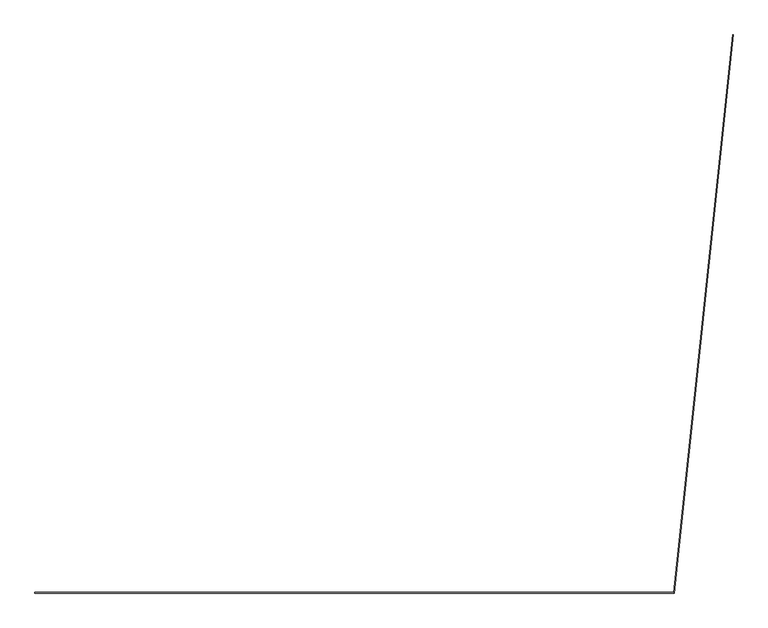
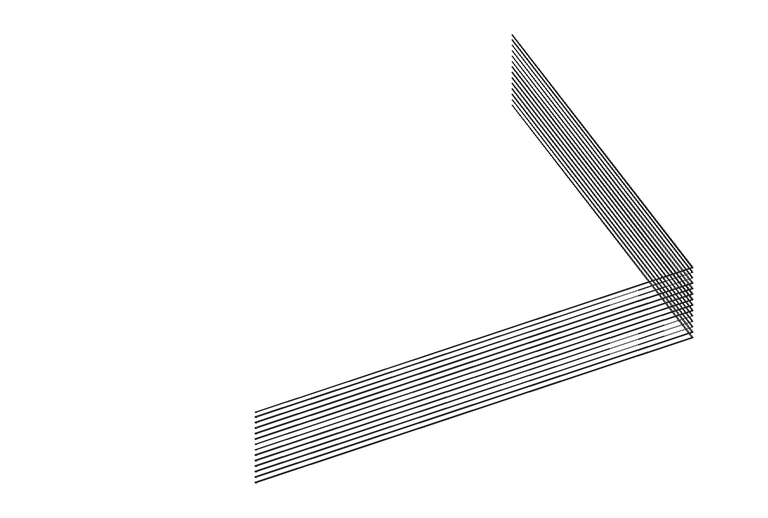
"""IFC4 building model written with IfcOpenShell, lengths in millimetres: railing geometry."""

import ifcopenshell
import ifcopenshell.guid

model = None  # the IFC model being written
_history = None  # IfcOwnerHistory: only IFC2X3 demands one
_inside = {}  # id of a spatial element -> (the spatial element, [elements in it])
_under = {}  # id of a project, library or spatial element -> (it, [spatial elements below it])
_declared = {}  # id of a project -> (the project, [libraries it declares])
_typed = {}  # id of a type object -> (the type object, [elements of that type])
_made_of = {}  # id of a material, layer set ... -> (it, [elements and type objects made of it])


def new_model(schema):
    """Start an empty IFC model of exactly this schema.

    Asked for "IFC4X3", IfcOpenShell would pick the latest addendum, in which some entities
    have other attributes; the version numbers below select the first issue.
    IFC2X3 requires an IfcOwnerHistory on every rooted entity: one is made here for all.
    """
    global model, _history
    if schema == "IFC4X3":
        model = ifcopenshell.file(schema_version=(4, 3, 0, 0))
    else:
        model = ifcopenshell.file(schema=schema)
    _inside.clear()
    _under.clear()
    _declared.clear()
    _typed.clear()
    _made_of.clear()
    _history = None
    if model.schema == "IFC2X3":
        org = make("IfcOrganization", Name="unknown")
        user = make(
            "IfcPersonAndOrganization",
            ThePerson=make("IfcPerson", FamilyName="unknown"),
            TheOrganization=org,
        )
        app = make(
            "IfcApplication",
            ApplicationDeveloper=org,
            Version="unknown",
            ApplicationFullName="unknown",
            ApplicationIdentifier="unknown",
        )
        _history = make(
            "IfcOwnerHistory",
            OwningUser=user,
            OwningApplication=app,
            ChangeAction="ADDED",
            CreationDate=0,
        )
    return model


def make(cls, **values):
    """One entity of the class cls with the attributes given. An attribute that is None is left unset."""
    return model.create_entity(
        cls, **{name: value for name, value in values.items() if value is not None}
    )


def rooted(cls, **values):
    """An entity with a GlobalId (a new one), such as an element, a storey or a relation."""
    return make(cls, GlobalId=ifcopenshell.guid.new(), OwnerHistory=_history, **values)


def si_unit(unit_type, name, prefix=None):
    """IfcSIUnit, for example si_unit("LENGTHUNIT", "METRE", prefix="MILLI")."""
    return make("IfcSIUnit", UnitType=unit_type, Prefix=prefix, Name=name)


def assignment(units):
    """IfcUnitAssignment: the units of a project."""
    return None if units is None else make("IfcUnitAssignment", Units=units)


def point(xyz):
    """IfcCartesianPoint."""
    return None if xyz is None else make("IfcCartesianPoint", Coordinates=xyz)


def direction(xyz):
    """IfcDirection."""
    return None if xyz is None else make("IfcDirection", DirectionRatios=xyz)


def frame(location, z_axis=None, x_axis=None):
    """IfcAxis2Placement3D, a coordinate frame: its origin and axes. An axis left out is left unset."""
    return make(
        "IfcAxis2Placement3D",
        Location=point(location),
        Axis=direction(z_axis),
        RefDirection=direction(x_axis),
    )


def origin():
    """The frame at (0, 0, 0) with its axes left unset."""
    return frame((0.0, 0.0, 0.0))


def place(relative_to, where):
    """IfcLocalPlacement: puts the frame where relative to a parent placement (None: the world)."""
    return make(
        "IfcLocalPlacement", PlacementRelTo=relative_to, RelativePlacement=where
    )


def context(
    kind, dimensions, precision=None, world=None, true_north=None, identifier=None
):
    """IfcGeometricRepresentationContext, for example the 3D "Model" context."""
    return make(
        "IfcGeometricRepresentationContext",
        ContextIdentifier=identifier,
        ContextType=kind,
        CoordinateSpaceDimension=dimensions,
        Precision=precision,
        WorldCoordinateSystem=world,
        TrueNorth=true_north,
    )


def project(units=None, contexts=None):
    """IfcProject with its units and contexts."""
    return rooted(
        "IfcProject",
        Name="project",
        RepresentationContexts=contexts,
        UnitsInContext=assignment(units),
    )


def spatial(cls, under=None, at=None, **own):
    """A site, building, storey or space (cls), placed at a placement, below another one or the project."""
    s = rooted(cls, ObjectPlacement=at, **own)
    if under is not None:
        _under.setdefault(under.id(), (under, []))[1].append(s)
    return s


def circle_curve(where, radius):
    """IfcCircle in the frame where."""
    return make("IfcCircle", Position=where, Radius=radius)


def ellipse_curve(where, semi_axis1, semi_axis2):
    """IfcEllipse in the frame where."""
    return make(
        "IfcEllipse", Position=where, SemiAxis1=semi_axis1, SemiAxis2=semi_axis2
    )


def shape(context_of_items, identifier, shape_type, items):
    """IfcShapeRepresentation: the items that make up one representation, for example the "Body"."""
    return make(
        "IfcShapeRepresentation",
        ContextOfItems=context_of_items,
        RepresentationIdentifier=identifier,
        RepresentationType=shape_type,
        Items=items,
    )


def source(mapping_origin, context_of_items, identifier, shape_type, items):
    """IfcRepresentationMap: a shape defined once, which mapped items show again and again."""
    return make(
        "IfcRepresentationMap",
        MappingOrigin=mapping_origin,
        MappedRepresentation=shape(context_of_items, identifier, shape_type, items),
    )


def transform(
    local_origin,
    x_axis=None,
    y_axis=None,
    z_axis=None,
    scale=None,
    scale2=None,
    scale3=None,
    uniform=True,
):
    """IfcCartesianTransformationOperator3D, or its non-uniform kind. x_axis, y_axis, z_axis: its Axis1, 2, 3."""
    if uniform:
        return make(
            "IfcCartesianTransformationOperator3D",
            Axis1=direction(x_axis),
            Axis2=direction(y_axis),
            LocalOrigin=point(local_origin),
            Scale=scale,
            Axis3=direction(z_axis),
        )
    return make(
        "IfcCartesianTransformationOperator3DnonUniform",
        Axis1=direction(x_axis),
        Axis2=direction(y_axis),
        LocalOrigin=point(local_origin),
        Scale=scale,
        Axis3=direction(z_axis),
        Scale2=scale2,
        Scale3=scale3,
    )


def mapped(mapping_source, mapping_target):
    """IfcMappedItem: shows the shape of a source again, moved by a transform."""
    return make(
        "IfcMappedItem", MappingSource=mapping_source, MappingTarget=mapping_target
    )


def made_of(thing, what):
    """Note that an element or type object is made of a material, layer set ...; save() writes the relation."""
    if what is not None:
        _made_of.setdefault(what.id(), (what, []))[1].append(thing)
    return thing


def element(
    cls,
    number,
    at=None,
    inside=None,
    cuts=None,
    type_object=None,
    material=None,
    context=None,
    identifier="Body",
    shape_type=None,
    held_by="IfcProductDefinitionShape",
    body=None,
    shapes=None,
    **own,
):
    """One element of the class cls, such as IfcWall. Its Tag is "e" and its number.

    at: its placement. inside: the storey or other place that contains it. cuts: it is an
    opening in that element (IfcRelVoidsElement). A single representation is given by context,
    identifier, shape_type and body (its items); several are given by shapes. held_by: the class
    of the entity that holds the representations. save() writes the other relations.
    """
    e = rooted(cls, Tag="e%d" % number, ObjectPlacement=at, **own)
    if body is not None:
        shapes = [shape(context, identifier, shape_type, body)]
    if shapes is not None:
        e.Representation = make(held_by, Representations=shapes)
    if inside is not None:
        _inside.setdefault(inside.id(), (inside, []))[1].append(e)
    if cuts is not None:
        rooted(
            "IfcRelVoidsElement", RelatingBuildingElement=cuts, RelatedOpeningElement=e
        )
    if type_object is not None:
        _typed.setdefault(type_object.id(), (type_object, []))[1].append(e)
    return made_of(e, material)


def aggregate(whole, parts):
    """IfcRelAggregates: a whole, such as a stair, and the parts it consists of."""
    return rooted("IfcRelAggregates", RelatingObject=whole, RelatedObjects=parts)


def save(model, path):
    """Write the relations noted so far, then the file.

    IfcRelAggregates (storeys below a building ...), IfcRelContainedInSpatialStructure (elements
    in a storey), IfcRelDefinesByType, IfcRelAssociatesMaterial and IfcRelDeclares: one each for
    every whole, place, type object, material and project.
    """
    for whole, parts in _under.values():
        aggregate(whole, parts)
    for where, things in _inside.values():
        rooted(
            "IfcRelContainedInSpatialStructure",
            RelatedElements=things,
            RelatingStructure=where,
        )
    for kind, things in _typed.values():
        rooted("IfcRelDefinesByType", RelatedObjects=things, RelatingType=kind)
    for what, things in _made_of.values():
        rooted("IfcRelAssociatesMaterial", RelatedObjects=things, RelatingMaterial=what)
    for by, libraries in _declared.values():
        rooted("IfcRelDeclares", RelatingContext=by, RelatedDefinitions=libraries)
    model.write(path)


def plane_surface(at):
    """IfcPlane: the flat surface through the origin of the frame at, square to its z axis."""
    return make("IfcPlane", Position=at)


def cylinder_surface(at, radius):
    """IfcCylindricalSurface: all points at the distance radius from the z axis of the frame at."""
    return make("IfcCylindricalSurface", Position=at, Radius=radius)


def advanced_brep(points, edges, surfaces, faces):
    """IfcAdvancedBrep: a solid bounded by faces that lie on surfaces and meet in shared edges.

    An edge is (start, end): straight between two places in points (the first is 0);
    or (start, end, curve); or (start, end, curve, False) where it runs against its curve.
    A face is (place in surfaces, loops), or (place, loops, False) where it looks against
    its surface's normal. A loop lists edges by number (the first is 1), with a minus sign
    where the edge is run from its end to its start. The first loop is the outer one.
    """
    corners = [point(p) for p in points]
    vertices = [make("IfcVertexPoint", VertexGeometry=c) for c in corners]
    made = []
    for start, end, *more in edges:
        made.append(
            make(
                "IfcEdgeCurve",
                EdgeStart=vertices[start],
                EdgeEnd=vertices[end],
                EdgeGeometry=more[0] if more else make("IfcPolyline", Points=[corners[start], corners[end]]),
                SameSense=more[1] if len(more) > 1 else True,
            )
        )
    hull = []
    for where, loops, *sense in faces:
        bounds = []
        for j, loop in enumerate(loops):
            ring = [make("IfcOrientedEdge", EdgeElement=made[abs(k) - 1], Orientation=k > 0) for k in loop]
            bounds.append(
                make(
                    "IfcFaceOuterBound" if j == 0 else "IfcFaceBound",
                    Bound=make("IfcEdgeLoop", EdgeList=ring),
                    Orientation=True,
                )
            )
        hull.append(make("IfcAdvancedFace", Bounds=bounds, FaceSurface=surfaces[where], SameSense=sense[0] if sense else True))
    return make("IfcAdvancedBrep", Outer=make("IfcClosedShell", CfsFaces=hull))


def railing_c9f429d1(model_context):
    return source(origin(), model_context, "Body", "AdvancedBrep", [
        advanced_brep(
        [(34239.1491327, 30677.9041051, 270256.79375), (34234.4127222, 30678.4019219, 270256.79375), (27919.3590778, 25622.1094112, 270256.79375), (27919.3590778, 25626.8719112, 270256.79375), (33707.7636978, 25622.1094112, 270256.79375), (33703.4755235, 25626.8719112, 270256.79375)],
        [
            (0, 1, circle_curve(frame((34236.7809275, 30678.1530135, 270256.79375), z_axis=(0.10452846326765991, 0.9945218953682727, 0.0), x_axis=(-0.9945218953682727, 0.10452846326765991, 0.0)), 2.38125)),
            (1, 0, circle_curve(frame((34236.7809275, 30678.1530135, 270256.79375), z_axis=(0.10452846326765991, 0.9945218953682727, 0.0), x_axis=(-0.9945218953682727, 0.10452846326765991, 0.0)), 2.38125)),
            (2, 3, circle_curve(frame((27919.3590778, 25624.4906612, 270256.79375), z_axis=(-1.0, 0.0, 0.0), x_axis=(0.0, 1.0, 0.0)), 2.38125)),
            (3, 2, circle_curve(frame((27919.3590778, 25624.4906612, 270256.79375), z_axis=(-1.0, 0.0, 0.0), x_axis=(0.0, 1.0, 0.0)), 2.38125)),
            (0, 4),
            (4, 5, ellipse_curve(frame((33705.6196106, 25624.4906612, 270256.79375), z_axis=(0.7431448254773977, 0.6691306063588546, 0.0), x_axis=(-0.6691306063588546, 0.7431448254773974, 0.0)), 3.2042879, 2.38125)),
            (5, 1),
            (5, 4, ellipse_curve(frame((33705.6196106, 25624.4906612, 270256.79375), z_axis=(0.7431448254773977, 0.6691306063588546, 0.0), x_axis=(-0.6691306063588546, 0.7431448254773974, 0.0)), 3.2042879, 2.38125)),
            (4, 2),
            (3, 5),
        ],
        [
            plane_surface(frame((34236.7809275, 30678.1530135, 270259.175), z_axis=(0.10452846326765991, 0.9945218953682727, 0.0), x_axis=(0.9945218953682727, -0.10452846326765991, 0.0))),
            plane_surface(frame((27919.3590778, 25624.4906612, 270259.175), z_axis=(-1.0, 0.0, 0.0), x_axis=(0.0, -1.0, 0.0))),
            cylinder_surface(frame((34236.7809275, 30678.1530135, 270256.79375), z_axis=(0.10452846326765991, 0.9945218953682727, 0.0), x_axis=(-0.9945218953682727, 0.10452846326765991, 0.0)), 2.38125),
            cylinder_surface(frame((33705.6196106, 25624.4906612, 270256.79375), z_axis=(1.0, 0.0, 0.0), x_axis=(0.0, 1.0, 0.0)), 2.38125),
        ],
        [
            (0, [[1, 2]]),
            (1, [[3, 4]]),
            (2, [[-1, 5, 6, 7]]),
            (2, [[-2, -7, 8, -5]]),
            (3, [[-6, 9, -4, 10]]),
            (3, [[-8, -10, -3, -9]]),
        ],
    ),
        advanced_brep(
        [(34239.1491327, 30677.9041051, 270190.11875), (34234.4127222, 30678.4019219, 270190.11875), (33707.7636978, 25622.1094112, 270190.11875), (33703.4755235, 25626.8719112, 270190.11875), (27919.3590778, 25622.1094112, 270190.11875), (27919.3590778, 25626.8719112, 270190.11875)],
        [
            (0, 1, circle_curve(frame((34236.7809275, 30678.1530135, 270190.11875), z_axis=(0.10452846326765991, 0.9945218953682727, 0.0), x_axis=(-0.9945218953682727, 0.10452846326765991, 0.0)), 2.38125)),
            (1, 0, circle_curve(frame((34236.7809275, 30678.1530135, 270190.11875), z_axis=(0.10452846326765991, 0.9945218953682727, 0.0), x_axis=(-0.9945218953682727, 0.10452846326765991, 0.0)), 2.38125)),
            (0, 2),
            (2, 3, ellipse_curve(frame((33705.6196106, 25624.4906612, 270190.11875), z_axis=(0.7431448254773977, 0.6691306063588546, 0.0), x_axis=(-0.6691306063588546, 0.7431448254773974, 0.0)), 3.2042879, 2.38125)),
            (3, 1),
            (3, 2, ellipse_curve(frame((33705.6196106, 25624.4906612, 270190.11875), z_axis=(0.7431448254773977, 0.6691306063588546, 0.0), x_axis=(-0.6691306063588546, 0.7431448254773974, 0.0)), 3.2042879, 2.38125)),
            (4, 5, circle_curve(frame((27919.3590778, 25624.4906612, 270190.11875), z_axis=(-1.0, 0.0, 0.0), x_axis=(0.0, 1.0, 0.0)), 2.38125)),
            (5, 4, circle_curve(frame((27919.3590778, 25624.4906612, 270190.11875), z_axis=(-1.0, 0.0, 0.0), x_axis=(0.0, 1.0, 0.0)), 2.38125)),
            (2, 4),
            (5, 3),
        ],
        [
            plane_surface(frame((34236.7809275, 30678.1530135, 270192.5), z_axis=(0.10452846326765991, 0.9945218953682727, 0.0), x_axis=(0.9945218953682727, -0.10452846326765991, 0.0))),
            cylinder_surface(frame((34236.7809275, 30678.1530135, 270190.11875), z_axis=(0.10452846326765991, 0.9945218953682727, 0.0), x_axis=(-0.9945218953682727, 0.10452846326765991, 0.0)), 2.38125),
            plane_surface(frame((27919.3590778, 25624.4906612, 270192.5), z_axis=(-1.0, 0.0, 0.0), x_axis=(0.0, -1.0, 0.0))),
            cylinder_surface(frame((33705.6196106, 25624.4906612, 270190.11875), z_axis=(1.0, 0.0, 0.0), x_axis=(0.0, 1.0, 0.0)), 2.38125),
        ],
        [
            (0, [[1, 2]]),
            (1, [[-1, 3, 4, 5]]),
            (1, [[-2, -5, 6, -3]]),
            (2, [[7, 8]]),
            (3, [[-4, 9, -8, 10]]),
            (3, [[-6, -10, -7, -9]]),
        ],
    ),
        advanced_brep(
        [(34239.1491327, 30677.9041051, 270113.91875), (34234.4127222, 30678.4019219, 270113.91875), (33707.7636978, 25622.1094112, 270113.91875), (33703.4755235, 25626.8719112, 270113.91875), (27919.3590778, 25622.1094112, 270113.91875), (27919.3590778, 25626.8719112, 270113.91875)],
        [
            (0, 1, circle_curve(frame((34236.7809275, 30678.1530135, 270113.91875), z_axis=(0.10452846326765991, 0.9945218953682727, 0.0), x_axis=(-0.9945218953682727, 0.10452846326765991, 0.0)), 2.38125)),
            (1, 0, circle_curve(frame((34236.7809275, 30678.1530135, 270113.91875), z_axis=(0.10452846326765991, 0.9945218953682727, 0.0), x_axis=(-0.9945218953682727, 0.10452846326765991, 0.0)), 2.38125)),
            (0, 2),
            (2, 3, ellipse_curve(frame((33705.6196106, 25624.4906612, 270113.91875), z_axis=(0.7431448254773977, 0.6691306063588546, 0.0), x_axis=(-0.6691306063588546, 0.7431448254773974, 0.0)), 3.2042879, 2.38125)),
            (3, 1),
            (3, 2, ellipse_curve(frame((33705.6196106, 25624.4906612, 270113.91875), z_axis=(0.7431448254773977, 0.6691306063588546, 0.0), x_axis=(-0.6691306063588546, 0.7431448254773974, 0.0)), 3.2042879, 2.38125)),
            (4, 5, circle_curve(frame((27919.3590778, 25624.4906612, 270113.91875), z_axis=(-1.0, 0.0, 0.0), x_axis=(0.0, 1.0, 0.0)), 2.38125)),
            (5, 4, circle_curve(frame((27919.3590778, 25624.4906612, 270113.91875), z_axis=(-1.0, 0.0, 0.0), x_axis=(0.0, 1.0, 0.0)), 2.38125)),
            (2, 4),
            (5, 3),
        ],
        [
            plane_surface(frame((34236.7809275, 30678.1530135, 270116.3), z_axis=(0.10452846326765991, 0.9945218953682727, 0.0), x_axis=(0.9945218953682727, -0.10452846326765991, 0.0))),
            cylinder_surface(frame((34236.7809275, 30678.1530135, 270113.91875), z_axis=(0.10452846326765991, 0.9945218953682727, 0.0), x_axis=(-0.9945218953682727, 0.10452846326765991, 0.0)), 2.38125),
            plane_surface(frame((27919.3590778, 25624.4906612, 270116.3), z_axis=(-1.0, 0.0, 0.0), x_axis=(0.0, -1.0, 0.0))),
            cylinder_surface(frame((33705.6196106, 25624.4906612, 270113.91875), z_axis=(1.0, 0.0, 0.0), x_axis=(0.0, 1.0, 0.0)), 2.38125),
        ],
        [
            (0, [[1, 2]]),
            (1, [[-1, 3, 4, 5]]),
            (1, [[-2, -5, 6, -3]]),
            (2, [[7, 8]]),
            (3, [[-4, 9, -8, 10]]),
            (3, [[-6, -10, -7, -9]]),
        ],
    ),
        advanced_brep(
        [(34239.1491327, 30677.9041051, 270037.71875), (34234.4127222, 30678.4019219, 270037.71875), (33707.7636978, 25622.1094112, 270037.71875), (33703.4755235, 25626.8719112, 270037.71875), (27919.3590778, 25622.1094112, 270037.71875), (27919.3590778, 25626.8719112, 270037.71875)],
        [
            (0, 1, circle_curve(frame((34236.7809275, 30678.1530135, 270037.71875), z_axis=(0.10452846326765991, 0.9945218953682727, 0.0), x_axis=(-0.9945218953682727, 0.10452846326765991, 0.0)), 2.38125)),
            (1, 0, circle_curve(frame((34236.7809275, 30678.1530135, 270037.71875), z_axis=(0.10452846326765991, 0.9945218953682727, 0.0), x_axis=(-0.9945218953682727, 0.10452846326765991, 0.0)), 2.38125)),
            (0, 2),
            (2, 3, ellipse_curve(frame((33705.6196106, 25624.4906612, 270037.71875), z_axis=(0.7431448254773977, 0.6691306063588546, 0.0), x_axis=(-0.6691306063588546, 0.7431448254773974, 0.0)), 3.2042879, 2.38125)),
            (3, 1),
            (3, 2, ellipse_curve(frame((33705.6196106, 25624.4906612, 270037.71875), z_axis=(0.7431448254773977, 0.6691306063588546, 0.0), x_axis=(-0.6691306063588546, 0.7431448254773974, 0.0)), 3.2042879, 2.38125)),
            (4, 5, circle_curve(frame((27919.3590778, 25624.4906612, 270037.71875), z_axis=(-1.0, 0.0, 0.0), x_axis=(0.0, 1.0, 0.0)), 2.38125)),
            (5, 4, circle_curve(frame((27919.3590778, 25624.4906612, 270037.71875), z_axis=(-1.0, 0.0, 0.0), x_axis=(0.0, 1.0, 0.0)), 2.38125)),
            (2, 4),
            (5, 3),
        ],
        [
            plane_surface(frame((34236.7809275, 30678.1530135, 270040.1), z_axis=(0.10452846326765991, 0.9945218953682727, 0.0), x_axis=(0.9945218953682727, -0.10452846326765991, 0.0))),
            cylinder_surface(frame((34236.7809275, 30678.1530135, 270037.71875), z_axis=(0.10452846326765991, 0.9945218953682727, 0.0), x_axis=(-0.9945218953682727, 0.10452846326765991, 0.0)), 2.38125),
            plane_surface(frame((27919.3590778, 25624.4906612, 270040.1), z_axis=(-1.0, 0.0, 0.0), x_axis=(0.0, -1.0, 0.0))),
            cylinder_surface(frame((33705.6196106, 25624.4906612, 270037.71875), z_axis=(1.0, 0.0, 0.0), x_axis=(0.0, 1.0, 0.0)), 2.38125),
        ],
        [
            (0, [[1, 2]]),
            (1, [[-1, 3, 4, 5]]),
            (1, [[-2, -5, 6, -3]]),
            (2, [[7, 8]]),
            (3, [[-4, 9, -8, 10]]),
            (3, [[-6, -10, -7, -9]]),
        ],
    ),
        advanced_brep(
        [(34239.1491327, 30677.9041051, 269961.51875), (34234.4127222, 30678.4019219, 269961.51875), (33707.7636978, 25622.1094112, 269961.51875), (33703.4755235, 25626.8719112, 269961.51875), (27919.3590778, 25622.1094112, 269961.51875), (27919.3590778, 25626.8719112, 269961.51875)],
        [
            (0, 1, circle_curve(frame((34236.7809275, 30678.1530135, 269961.51875), z_axis=(0.10452846326765991, 0.9945218953682727, 0.0), x_axis=(-0.9945218953682727, 0.10452846326765991, 0.0)), 2.38125)),
            (1, 0, circle_curve(frame((34236.7809275, 30678.1530135, 269961.51875), z_axis=(0.10452846326765991, 0.9945218953682727, 0.0), x_axis=(-0.9945218953682727, 0.10452846326765991, 0.0)), 2.38125)),
            (0, 2),
            (2, 3, ellipse_curve(frame((33705.6196106, 25624.4906612, 269961.51875), z_axis=(0.7431448254773977, 0.6691306063588546, 0.0), x_axis=(-0.6691306063588546, 0.7431448254773974, 0.0)), 3.2042879, 2.38125)),
            (3, 1),
            (3, 2, ellipse_curve(frame((33705.6196106, 25624.4906612, 269961.51875), z_axis=(0.7431448254773977, 0.6691306063588546, 0.0), x_axis=(-0.6691306063588546, 0.7431448254773974, 0.0)), 3.2042879, 2.38125)),
            (4, 5, circle_curve(frame((27919.3590778, 25624.4906612, 269961.51875), z_axis=(-1.0, 0.0, 0.0), x_axis=(0.0, 1.0, 0.0)), 2.38125)),
            (5, 4, circle_curve(frame((27919.3590778, 25624.4906612, 269961.51875), z_axis=(-1.0, 0.0, 0.0), x_axis=(0.0, 1.0, 0.0)), 2.38125)),
            (2, 4),
            (5, 3),
        ],
        [
            plane_surface(frame((34236.7809275, 30678.1530135, 269963.9), z_axis=(0.10452846326765991, 0.9945218953682727, 0.0), x_axis=(0.9945218953682727, -0.10452846326765991, 0.0))),
            cylinder_surface(frame((34236.7809275, 30678.1530135, 269961.51875), z_axis=(0.10452846326765991, 0.9945218953682727, 0.0), x_axis=(-0.9945218953682727, 0.10452846326765991, 0.0)), 2.38125),
            plane_surface(frame((27919.3590778, 25624.4906612, 269963.9), z_axis=(-1.0, 0.0, 0.0), x_axis=(0.0, -1.0, 0.0))),
            cylinder_surface(frame((33705.6196106, 25624.4906612, 269961.51875), z_axis=(1.0, 0.0, 0.0), x_axis=(0.0, 1.0, 0.0)), 2.38125),
        ],
        [
            (0, [[1, 2]]),
            (1, [[-1, 3, 4, 5]]),
            (1, [[-2, -5, 6, -3]]),
            (2, [[7, 8]]),
            (3, [[-4, 9, -8, 10]]),
            (3, [[-6, -10, -7, -9]]),
        ],
    ),
        advanced_brep(
        [(34239.1491327, 30677.9041051, 269885.31875), (34234.4127222, 30678.4019219, 269885.31875), (33707.7636978, 25622.1094112, 269885.31875), (33703.4755235, 25626.8719112, 269885.31875), (27919.3590778, 25622.1094112, 269885.31875), (27919.3590778, 25626.8719112, 269885.31875)],
        [
            (0, 1, circle_curve(frame((34236.7809275, 30678.1530135, 269885.31875), z_axis=(0.10452846326765991, 0.9945218953682727, 0.0), x_axis=(-0.9945218953682727, 0.10452846326765991, 0.0)), 2.38125)),
            (1, 0, circle_curve(frame((34236.7809275, 30678.1530135, 269885.31875), z_axis=(0.10452846326765991, 0.9945218953682727, 0.0), x_axis=(-0.9945218953682727, 0.10452846326765991, 0.0)), 2.38125)),
            (0, 2),
            (2, 3, ellipse_curve(frame((33705.6196106, 25624.4906612, 269885.31875), z_axis=(0.7431448254773977, 0.6691306063588546, 0.0), x_axis=(-0.6691306063588546, 0.7431448254773974, 0.0)), 3.2042879, 2.38125)),
            (3, 1),
            (3, 2, ellipse_curve(frame((33705.6196106, 25624.4906612, 269885.31875), z_axis=(0.7431448254773977, 0.6691306063588546, 0.0), x_axis=(-0.6691306063588546, 0.7431448254773974, 0.0)), 3.2042879, 2.38125)),
            (4, 5, circle_curve(frame((27919.3590778, 25624.4906612, 269885.31875), z_axis=(-1.0, 0.0, 0.0), x_axis=(0.0, 1.0, 0.0)), 2.38125)),
            (5, 4, circle_curve(frame((27919.3590778, 25624.4906612, 269885.31875), z_axis=(-1.0, 0.0, 0.0), x_axis=(0.0, 1.0, 0.0)), 2.38125)),
            (2, 4),
            (5, 3),
        ],
        [
            plane_surface(frame((34236.7809275, 30678.1530135, 269887.7), z_axis=(0.10452846326765991, 0.9945218953682727, 0.0), x_axis=(0.9945218953682727, -0.10452846326765991, 0.0))),
            cylinder_surface(frame((34236.7809275, 30678.1530135, 269885.31875), z_axis=(0.10452846326765991, 0.9945218953682727, 0.0), x_axis=(-0.9945218953682727, 0.10452846326765991, 0.0)), 2.38125),
            plane_surface(frame((27919.3590778, 25624.4906612, 269887.7), z_axis=(-1.0, 0.0, 0.0), x_axis=(0.0, -1.0, 0.0))),
            cylinder_surface(frame((33705.6196106, 25624.4906612, 269885.31875), z_axis=(1.0, 0.0, 0.0), x_axis=(0.0, 1.0, 0.0)), 2.38125),
        ],
        [
            (0, [[1, 2]]),
            (1, [[-1, 3, 4, 5]]),
            (1, [[-2, -5, 6, -3]]),
            (2, [[7, 8]]),
            (3, [[-4, 9, -8, 10]]),
            (3, [[-6, -10, -7, -9]]),
        ],
    ),
        advanced_brep(
        [(34239.1491327, 30677.9041051, 269809.11875), (34234.4127222, 30678.4019219, 269809.11875), (33707.7636978, 25622.1094112, 269809.11875), (33703.4755235, 25626.8719112, 269809.11875), (27919.3590778, 25622.1094112, 269809.11875), (27919.3590778, 25626.8719112, 269809.11875)],
        [
            (0, 1, circle_curve(frame((34236.7809275, 30678.1530135, 269809.11875), z_axis=(0.10452846326765991, 0.9945218953682727, 0.0), x_axis=(-0.9945218953682727, 0.10452846326765991, 0.0)), 2.38125)),
            (1, 0, circle_curve(frame((34236.7809275, 30678.1530135, 269809.11875), z_axis=(0.10452846326765991, 0.9945218953682727, 0.0), x_axis=(-0.9945218953682727, 0.10452846326765991, 0.0)), 2.38125)),
            (0, 2),
            (2, 3, ellipse_curve(frame((33705.6196106, 25624.4906612, 269809.11875), z_axis=(0.7431448254773977, 0.6691306063588546, 0.0), x_axis=(-0.6691306063588546, 0.7431448254773974, 0.0)), 3.2042879, 2.38125)),
            (3, 1),
            (3, 2, ellipse_curve(frame((33705.6196106, 25624.4906612, 269809.11875), z_axis=(0.7431448254773977, 0.6691306063588546, 0.0), x_axis=(-0.6691306063588546, 0.7431448254773974, 0.0)), 3.2042879, 2.38125)),
            (4, 5, circle_curve(frame((27919.3590778, 25624.4906612, 269809.11875), z_axis=(-1.0, 0.0, 0.0), x_axis=(0.0, 1.0, 0.0)), 2.38125)),
            (5, 4, circle_curve(frame((27919.3590778, 25624.4906612, 269809.11875), z_axis=(-1.0, 0.0, 0.0), x_axis=(0.0, 1.0, 0.0)), 2.38125)),
            (2, 4),
            (5, 3),
        ],
        [
            plane_surface(frame((34236.7809275, 30678.1530135, 269811.5), z_axis=(0.10452846326765991, 0.9945218953682727, 0.0), x_axis=(0.9945218953682727, -0.10452846326765991, 0.0))),
            cylinder_surface(frame((34236.7809275, 30678.1530135, 269809.11875), z_axis=(0.10452846326765991, 0.9945218953682727, 0.0), x_axis=(-0.9945218953682727, 0.10452846326765991, 0.0)), 2.38125),
            plane_surface(frame((27919.3590778, 25624.4906612, 269811.5), z_axis=(-1.0, 0.0, 0.0), x_axis=(0.0, -1.0, 0.0))),
            cylinder_surface(frame((33705.6196106, 25624.4906612, 269809.11875), z_axis=(1.0, 0.0, 0.0), x_axis=(0.0, 1.0, 0.0)), 2.38125),
        ],
        [
            (0, [[1, 2]]),
            (1, [[-1, 3, 4, 5]]),
            (1, [[-2, -5, 6, -3]]),
            (2, [[7, 8]]),
            (3, [[-4, 9, -8, 10]]),
            (3, [[-6, -10, -7, -9]]),
        ],
    ),
        advanced_brep(
        [(34239.1491327, 30677.9041051, 269732.91875), (34234.4127222, 30678.4019219, 269732.91875), (33707.7636978, 25622.1094112, 269732.91875), (33703.4755235, 25626.8719112, 269732.91875), (27919.3590778, 25622.1094112, 269732.91875), (27919.3590778, 25626.8719112, 269732.91875)],
        [
            (0, 1, circle_curve(frame((34236.7809275, 30678.1530135, 269732.91875), z_axis=(0.10452846326765991, 0.9945218953682727, 0.0), x_axis=(-0.9945218953682727, 0.10452846326765991, 0.0)), 2.38125)),
            (1, 0, circle_curve(frame((34236.7809275, 30678.1530135, 269732.91875), z_axis=(0.10452846326765991, 0.9945218953682727, 0.0), x_axis=(-0.9945218953682727, 0.10452846326765991, 0.0)), 2.38125)),
            (0, 2),
            (2, 3, ellipse_curve(frame((33705.6196106, 25624.4906612, 269732.91875), z_axis=(0.7431448254773977, 0.6691306063588546, 0.0), x_axis=(-0.6691306063588546, 0.7431448254773974, 0.0)), 3.2042879, 2.38125)),
            (3, 1),
            (3, 2, ellipse_curve(frame((33705.6196106, 25624.4906612, 269732.91875), z_axis=(0.7431448254773977, 0.6691306063588546, 0.0), x_axis=(-0.6691306063588546, 0.7431448254773974, 0.0)), 3.2042879, 2.38125)),
            (4, 5, circle_curve(frame((27919.3590778, 25624.4906612, 269732.91875), z_axis=(-1.0, 0.0, 0.0), x_axis=(0.0, 1.0, 0.0)), 2.38125)),
            (5, 4, circle_curve(frame((27919.3590778, 25624.4906612, 269732.91875), z_axis=(-1.0, 0.0, 0.0), x_axis=(0.0, 1.0, 0.0)), 2.38125)),
            (2, 4),
            (5, 3),
        ],
        [
            plane_surface(frame((34236.7809275, 30678.1530135, 269735.3), z_axis=(0.10452846326765991, 0.9945218953682727, 0.0), x_axis=(0.9945218953682727, -0.10452846326765991, 0.0))),
            cylinder_surface(frame((34236.7809275, 30678.1530135, 269732.91875), z_axis=(0.10452846326765991, 0.9945218953682727, 0.0), x_axis=(-0.9945218953682727, 0.10452846326765991, 0.0)), 2.38125),
            plane_surface(frame((27919.3590778, 25624.4906612, 269735.3), z_axis=(-1.0, 0.0, 0.0), x_axis=(0.0, -1.0, 0.0))),
            cylinder_surface(frame((33705.6196106, 25624.4906612, 269732.91875), z_axis=(1.0, 0.0, 0.0), x_axis=(0.0, 1.0, 0.0)), 2.38125),
        ],
        [
            (0, [[1, 2]]),
            (1, [[-1, 3, 4, 5]]),
            (1, [[-2, -5, 6, -3]]),
            (2, [[7, 8]]),
            (3, [[-4, 9, -8, 10]]),
            (3, [[-6, -10, -7, -9]]),
        ],
    ),
        advanced_brep(
        [(34239.1491327, 30677.9041051, 269656.71875), (34234.4127222, 30678.4019219, 269656.71875), (33707.7636978, 25622.1094112, 269656.71875), (33703.4755235, 25626.8719112, 269656.71875), (27919.3590778, 25622.1094112, 269656.71875), (27919.3590778, 25626.8719112, 269656.71875)],
        [
            (0, 1, circle_curve(frame((34236.7809275, 30678.1530135, 269656.71875), z_axis=(0.10452846326765991, 0.9945218953682727, 0.0), x_axis=(-0.9945218953682727, 0.10452846326765991, 0.0)), 2.38125)),
            (1, 0, circle_curve(frame((34236.7809275, 30678.1530135, 269656.71875), z_axis=(0.10452846326765991, 0.9945218953682727, 0.0), x_axis=(-0.9945218953682727, 0.10452846326765991, 0.0)), 2.38125)),
            (0, 2),
            (2, 3, ellipse_curve(frame((33705.6196106, 25624.4906612, 269656.71875), z_axis=(0.7431448254773977, 0.6691306063588546, 0.0), x_axis=(-0.6691306063588546, 0.7431448254773974, 0.0)), 3.2042879, 2.38125)),
            (3, 1),
            (3, 2, ellipse_curve(frame((33705.6196106, 25624.4906612, 269656.71875), z_axis=(0.7431448254773977, 0.6691306063588546, 0.0), x_axis=(-0.6691306063588546, 0.7431448254773974, 0.0)), 3.2042879, 2.38125)),
            (4, 5, circle_curve(frame((27919.3590778, 25624.4906612, 269656.71875), z_axis=(-1.0, 0.0, 0.0), x_axis=(0.0, 1.0, 0.0)), 2.38125)),
            (5, 4, circle_curve(frame((27919.3590778, 25624.4906612, 269656.71875), z_axis=(-1.0, 0.0, 0.0), x_axis=(0.0, 1.0, 0.0)), 2.38125)),
            (2, 4),
            (5, 3),
        ],
        [
            plane_surface(frame((34236.7809275, 30678.1530135, 269659.1), z_axis=(0.10452846326765991, 0.9945218953682727, 0.0), x_axis=(0.9945218953682727, -0.10452846326765991, 0.0))),
            cylinder_surface(frame((34236.7809275, 30678.1530135, 269656.71875), z_axis=(0.10452846326765991, 0.9945218953682727, 0.0), x_axis=(-0.9945218953682727, 0.10452846326765991, 0.0)), 2.38125),
            plane_surface(frame((27919.3590778, 25624.4906612, 269659.1), z_axis=(-1.0, 0.0, 0.0), x_axis=(0.0, -1.0, 0.0))),
            cylinder_surface(frame((33705.6196106, 25624.4906612, 269656.71875), z_axis=(1.0, 0.0, 0.0), x_axis=(0.0, 1.0, 0.0)), 2.38125),
        ],
        [
            (0, [[1, 2]]),
            (1, [[-1, 3, 4, 5]]),
            (1, [[-2, -5, 6, -3]]),
            (2, [[7, 8]]),
            (3, [[-4, 9, -8, 10]]),
            (3, [[-6, -10, -7, -9]]),
        ],
    ),
        advanced_brep(
        [(34239.1491327, 30677.9041051, 269580.51875), (34234.4127222, 30678.4019219, 269580.51875), (33707.7636978, 25622.1094112, 269580.51875), (33703.4755235, 25626.8719112, 269580.51875), (27919.3590778, 25622.1094112, 269580.51875), (27919.3590778, 25626.8719112, 269580.51875)],
        [
            (0, 1, circle_curve(frame((34236.7809275, 30678.1530135, 269580.51875), z_axis=(0.10452846326765991, 0.9945218953682727, 0.0), x_axis=(-0.9945218953682727, 0.10452846326765991, 0.0)), 2.38125)),
            (1, 0, circle_curve(frame((34236.7809275, 30678.1530135, 269580.51875), z_axis=(0.10452846326765991, 0.9945218953682727, 0.0), x_axis=(-0.9945218953682727, 0.10452846326765991, 0.0)), 2.38125)),
            (0, 2),
            (2, 3, ellipse_curve(frame((33705.6196106, 25624.4906612, 269580.51875), z_axis=(0.7431448254773977, 0.6691306063588546, 0.0), x_axis=(-0.6691306063588546, 0.7431448254773974, 0.0)), 3.2042879, 2.38125)),
            (3, 1),
            (3, 2, ellipse_curve(frame((33705.6196106, 25624.4906612, 269580.51875), z_axis=(0.7431448254773977, 0.6691306063588546, 0.0), x_axis=(-0.6691306063588546, 0.7431448254773974, 0.0)), 3.2042879, 2.38125)),
            (4, 5, circle_curve(frame((27919.3590778, 25624.4906612, 269580.51875), z_axis=(-1.0, 0.0, 0.0), x_axis=(0.0, 1.0, 0.0)), 2.38125)),
            (5, 4, circle_curve(frame((27919.3590778, 25624.4906612, 269580.51875), z_axis=(-1.0, 0.0, 0.0), x_axis=(0.0, 1.0, 0.0)), 2.38125)),
            (2, 4),
            (5, 3),
        ],
        [
            plane_surface(frame((34236.7809275, 30678.1530135, 269582.9), z_axis=(0.10452846326765991, 0.9945218953682727, 0.0), x_axis=(0.9945218953682727, -0.10452846326765991, 0.0))),
            cylinder_surface(frame((34236.7809275, 30678.1530135, 269580.51875), z_axis=(0.10452846326765991, 0.9945218953682727, 0.0), x_axis=(-0.9945218953682727, 0.10452846326765991, 0.0)), 2.38125),
            plane_surface(frame((27919.3590778, 25624.4906612, 269582.9), z_axis=(-1.0, 0.0, 0.0), x_axis=(0.0, -1.0, 0.0))),
            cylinder_surface(frame((33705.6196106, 25624.4906612, 269580.51875), z_axis=(1.0, 0.0, 0.0), x_axis=(0.0, 1.0, 0.0)), 2.38125),
        ],
        [
            (0, [[1, 2]]),
            (1, [[-1, 3, 4, 5]]),
            (1, [[-2, -5, 6, -3]]),
            (2, [[7, 8]]),
            (3, [[-4, 9, -8, 10]]),
            (3, [[-6, -10, -7, -9]]),
        ],
    ),
        advanced_brep(
        [(34239.1491327, 30677.9041051, 269504.31875), (34234.4127222, 30678.4019219, 269504.31875), (33707.7636978, 25622.1094112, 269504.31875), (33703.4755235, 25626.8719112, 269504.31875), (27919.3590778, 25622.1094112, 269504.31875), (27919.3590778, 25626.8719112, 269504.31875)],
        [
            (0, 1, circle_curve(frame((34236.7809275, 30678.1530135, 269504.31875), z_axis=(0.10452846326765991, 0.9945218953682727, 0.0), x_axis=(-0.9945218953682727, 0.10452846326765991, 0.0)), 2.38125)),
            (1, 0, circle_curve(frame((34236.7809275, 30678.1530135, 269504.31875), z_axis=(0.10452846326765991, 0.9945218953682727, 0.0), x_axis=(-0.9945218953682727, 0.10452846326765991, 0.0)), 2.38125)),
            (0, 2),
            (2, 3, ellipse_curve(frame((33705.6196106, 25624.4906612, 269504.31875), z_axis=(0.7431448254773977, 0.6691306063588546, 0.0), x_axis=(-0.6691306063588546, 0.7431448254773974, 0.0)), 3.2042879, 2.38125)),
            (3, 1),
            (3, 2, ellipse_curve(frame((33705.6196106, 25624.4906612, 269504.31875), z_axis=(0.7431448254773977, 0.6691306063588546, 0.0), x_axis=(-0.6691306063588546, 0.7431448254773974, 0.0)), 3.2042879, 2.38125)),
            (4, 5, circle_curve(frame((27919.3590778, 25624.4906612, 269504.31875), z_axis=(-1.0, 0.0, 0.0), x_axis=(0.0, 1.0, 0.0)), 2.38125)),
            (5, 4, circle_curve(frame((27919.3590778, 25624.4906612, 269504.31875), z_axis=(-1.0, 0.0, 0.0), x_axis=(0.0, 1.0, 0.0)), 2.38125)),
            (2, 4),
            (5, 3),
        ],
        [
            plane_surface(frame((34236.7809275, 30678.1530135, 269506.7), z_axis=(0.10452846326765991, 0.9945218953682727, 0.0), x_axis=(0.9945218953682727, -0.10452846326765991, 0.0))),
            cylinder_surface(frame((34236.7809275, 30678.1530135, 269504.31875), z_axis=(0.10452846326765991, 0.9945218953682727, 0.0), x_axis=(-0.9945218953682727, 0.10452846326765991, 0.0)), 2.38125),
            plane_surface(frame((27919.3590778, 25624.4906612, 269506.7), z_axis=(-1.0, 0.0, 0.0), x_axis=(0.0, -1.0, 0.0))),
            cylinder_surface(frame((33705.6196106, 25624.4906612, 269504.31875), z_axis=(1.0, 0.0, 0.0), x_axis=(0.0, 1.0, 0.0)), 2.38125),
        ],
        [
            (0, [[1, 2]]),
            (1, [[-1, 3, 4, 5]]),
            (1, [[-2, -5, 6, -3]]),
            (2, [[7, 8]]),
            (3, [[-4, 9, -8, 10]]),
            (3, [[-6, -10, -7, -9]]),
        ],
    ),
        advanced_brep(
        [(34239.1491327, 30677.9041051, 269428.11875), (34234.4127222, 30678.4019219, 269428.11875), (33707.7636978, 25622.1094112, 269428.11875), (33703.4755235, 25626.8719112, 269428.11875), (27919.3590778, 25622.1094112, 269428.11875), (27919.3590778, 25626.8719112, 269428.11875)],
        [
            (0, 1, circle_curve(frame((34236.7809275, 30678.1530135, 269428.11875), z_axis=(0.10452846326765991, 0.9945218953682727, 0.0), x_axis=(-0.9945218953682727, 0.10452846326765991, 0.0)), 2.38125)),
            (1, 0, circle_curve(frame((34236.7809275, 30678.1530135, 269428.11875), z_axis=(0.10452846326765991, 0.9945218953682727, 0.0), x_axis=(-0.9945218953682727, 0.10452846326765991, 0.0)), 2.38125)),
            (0, 2),
            (2, 3, ellipse_curve(frame((33705.6196106, 25624.4906612, 269428.11875), z_axis=(0.7431448254773977, 0.6691306063588546, 0.0), x_axis=(-0.6691306063588546, 0.7431448254773974, 0.0)), 3.2042879, 2.38125)),
            (3, 1),
            (3, 2, ellipse_curve(frame((33705.6196106, 25624.4906612, 269428.11875), z_axis=(0.7431448254773977, 0.6691306063588546, 0.0), x_axis=(-0.6691306063588546, 0.7431448254773974, 0.0)), 3.2042879, 2.38125)),
            (4, 5, circle_curve(frame((27919.3590778, 25624.4906612, 269428.11875), z_axis=(-1.0, 0.0, 0.0), x_axis=(0.0, 1.0, 0.0)), 2.38125)),
            (5, 4, circle_curve(frame((27919.3590778, 25624.4906612, 269428.11875), z_axis=(-1.0, 0.0, 0.0), x_axis=(0.0, 1.0, 0.0)), 2.38125)),
            (2, 4),
            (5, 3),
        ],
        [
            plane_surface(frame((34236.7809275, 30678.1530135, 269430.5), z_axis=(0.10452846326765991, 0.9945218953682727, 0.0), x_axis=(0.9945218953682727, -0.10452846326765991, 0.0))),
            cylinder_surface(frame((34236.7809275, 30678.1530135, 269428.11875), z_axis=(0.10452846326765991, 0.9945218953682727, 0.0), x_axis=(-0.9945218953682727, 0.10452846326765991, 0.0)), 2.38125),
            plane_surface(frame((27919.3590778, 25624.4906612, 269430.5), z_axis=(-1.0, 0.0, 0.0), x_axis=(0.0, -1.0, 0.0))),
            cylinder_surface(frame((33705.6196106, 25624.4906612, 269428.11875), z_axis=(1.0, 0.0, 0.0), x_axis=(0.0, 1.0, 0.0)), 2.38125),
        ],
        [
            (0, [[1, 2]]),
            (1, [[-1, 3, 4, 5]]),
            (1, [[-2, -5, 6, -3]]),
            (2, [[7, 8]]),
            (3, [[-4, 9, -8, 10]]),
            (3, [[-6, -10, -7, -9]]),
        ],
    ),
        advanced_brep(
        [(34239.1491327, 30677.9041051, 269351.91875), (34234.4127222, 30678.4019219, 269351.91875), (33707.7636978, 25622.1094112, 269351.91875), (33703.4755235, 25626.8719112, 269351.91875), (27919.3590778, 25622.1094112, 269351.91875), (27919.3590778, 25626.8719112, 269351.91875)],
        [
            (0, 1, circle_curve(frame((34236.7809275, 30678.1530135, 269351.91875), z_axis=(0.10452846326765991, 0.9945218953682727, 0.0), x_axis=(-0.9945218953682727, 0.10452846326765991, 0.0)), 2.38125)),
            (1, 0, circle_curve(frame((34236.7809275, 30678.1530135, 269351.91875), z_axis=(0.10452846326765991, 0.9945218953682727, 0.0), x_axis=(-0.9945218953682727, 0.10452846326765991, 0.0)), 2.38125)),
            (0, 2),
            (2, 3, ellipse_curve(frame((33705.6196106, 25624.4906612, 269351.91875), z_axis=(0.7431448254773977, 0.6691306063588546, 0.0), x_axis=(-0.6691306063588546, 0.7431448254773974, 0.0)), 3.2042879, 2.38125)),
            (3, 1),
            (3, 2, ellipse_curve(frame((33705.6196106, 25624.4906612, 269351.91875), z_axis=(0.7431448254773977, 0.6691306063588546, 0.0), x_axis=(-0.6691306063588546, 0.7431448254773974, 0.0)), 3.2042879, 2.38125)),
            (4, 5, circle_curve(frame((27919.3590778, 25624.4906612, 269351.91875), z_axis=(-1.0, 0.0, 0.0), x_axis=(0.0, 1.0, 0.0)), 2.38125)),
            (5, 4, circle_curve(frame((27919.3590778, 25624.4906612, 269351.91875), z_axis=(-1.0, 0.0, 0.0), x_axis=(0.0, 1.0, 0.0)), 2.38125)),
            (2, 4),
            (5, 3),
        ],
        [
            plane_surface(frame((34236.7809275, 30678.1530135, 269354.3), z_axis=(0.10452846326765991, 0.9945218953682727, 0.0), x_axis=(0.9945218953682727, -0.10452846326765991, 0.0))),
            cylinder_surface(frame((34236.7809275, 30678.1530135, 269351.91875), z_axis=(0.10452846326765991, 0.9945218953682727, 0.0), x_axis=(-0.9945218953682727, 0.10452846326765991, 0.0)), 2.38125),
            plane_surface(frame((27919.3590778, 25624.4906612, 269354.3), z_axis=(-1.0, 0.0, 0.0), x_axis=(0.0, -1.0, 0.0))),
            cylinder_surface(frame((33705.6196106, 25624.4906612, 269351.91875), z_axis=(1.0, 0.0, 0.0), x_axis=(0.0, 1.0, 0.0)), 2.38125),
        ],
        [
            (0, [[1, 2]]),
            (1, [[-1, 3, 4, 5]]),
            (1, [[-2, -5, 6, -3]]),
            (2, [[7, 8]]),
            (3, [[-4, 9, -8, 10]]),
            (3, [[-6, -10, -7, -9]]),
        ],
    ),
        advanced_brep(
        [(34239.1491327, 30677.9041051, 269275.71875), (34234.4127222, 30678.4019219, 269275.71875), (33707.7636978, 25622.1094112, 269275.71875), (33703.4755235, 25626.8719112, 269275.71875), (27919.3590778, 25622.1094112, 269275.71875), (27919.3590778, 25626.8719112, 269275.71875)],
        [
            (0, 1, circle_curve(frame((34236.7809275, 30678.1530135, 269275.71875), z_axis=(0.10452846326765991, 0.9945218953682727, 0.0), x_axis=(-0.9945218953682727, 0.10452846326765991, 0.0)), 2.38125)),
            (1, 0, circle_curve(frame((34236.7809275, 30678.1530135, 269275.71875), z_axis=(0.10452846326765991, 0.9945218953682727, 0.0), x_axis=(-0.9945218953682727, 0.10452846326765991, 0.0)), 2.38125)),
            (0, 2),
            (2, 3, ellipse_curve(frame((33705.6196106, 25624.4906612, 269275.71875), z_axis=(0.7431448254773977, 0.6691306063588546, 0.0), x_axis=(-0.6691306063588546, 0.7431448254773974, 0.0)), 3.2042879, 2.38125)),
            (3, 1),
            (3, 2, ellipse_curve(frame((33705.6196106, 25624.4906612, 269275.71875), z_axis=(0.7431448254773977, 0.6691306063588546, 0.0), x_axis=(-0.6691306063588546, 0.7431448254773974, 0.0)), 3.2042879, 2.38125)),
            (4, 5, circle_curve(frame((27919.3590778, 25624.4906612, 269275.71875), z_axis=(-1.0, 0.0, 0.0), x_axis=(0.0, 1.0, 0.0)), 2.38125)),
            (5, 4, circle_curve(frame((27919.3590778, 25624.4906612, 269275.71875), z_axis=(-1.0, 0.0, 0.0), x_axis=(0.0, 1.0, 0.0)), 2.38125)),
            (2, 4),
            (5, 3),
        ],
        [
            plane_surface(frame((34236.7809275, 30678.1530135, 269278.1), z_axis=(0.10452846326765991, 0.9945218953682727, 0.0), x_axis=(0.9945218953682727, -0.10452846326765991, 0.0))),
            cylinder_surface(frame((34236.7809275, 30678.1530135, 269275.71875), z_axis=(0.10452846326765991, 0.9945218953682727, 0.0), x_axis=(-0.9945218953682727, 0.10452846326765991, 0.0)), 2.38125),
            plane_surface(frame((27919.3590778, 25624.4906612, 269278.1), z_axis=(-1.0, 0.0, 0.0), x_axis=(0.0, -1.0, 0.0))),
            cylinder_surface(frame((33705.6196106, 25624.4906612, 269275.71875), z_axis=(1.0, 0.0, 0.0), x_axis=(0.0, 1.0, 0.0)), 2.38125),
        ],
        [
            (0, [[1, 2]]),
            (1, [[-1, 3, 4, 5]]),
            (1, [[-2, -5, 6, -3]]),
            (2, [[7, 8]]),
            (3, [[-4, 9, -8, 10]]),
            (3, [[-6, -10, -7, -9]]),
        ],
    ),
    ])


if __name__ == "__main__":
    model = new_model("IFC4")
    model_context = context("Model", 3, world=origin())
    ifc_project = project(units=[si_unit("LENGTHUNIT", "METRE", prefix="MILLI")], contexts=[model_context])
    site = spatial("IfcSite", under=ifc_project)
    building = spatial("IfcBuilding", under=site)
    placement = place(None, origin())
    railing_shape = railing_c9f429d1(model_context)
    element("IfcRailing", 1, at=placement, inside=building, context=model_context, shape_type="MappedRepresentation", body=[
        mapped(railing_shape, transform((0.0, 0.0, 0.0), x_axis=(1.0, 0.0, 0.0), y_axis=(0.0, 1.0, 0.0), z_axis=(0.0, 0.0, 1.0))),
    ])
    save(model, "model.ifc")

# Revit data of these elements
# Element 1 (IfcRailing)
#   Materials on its faces: "WIRE RAILING"
# Materials
#   "WIRE RAILING": class "Metal", colour RGB 244 244 244, transparency 0, Manufacturer = "Kawneer", URL = "http://www.kawneer.com/kawneer/north_america/en/home.asp", Cost = 0
